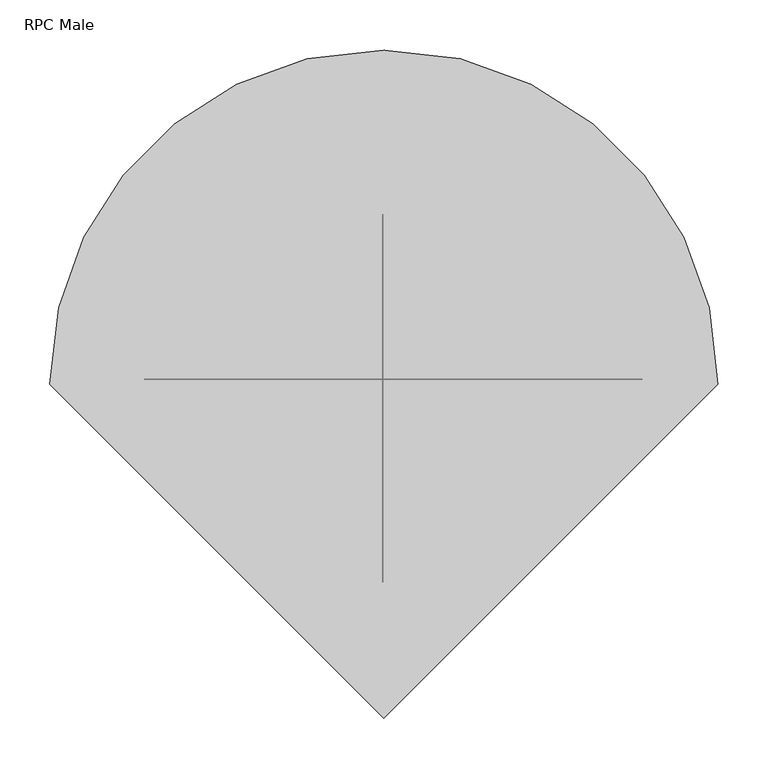
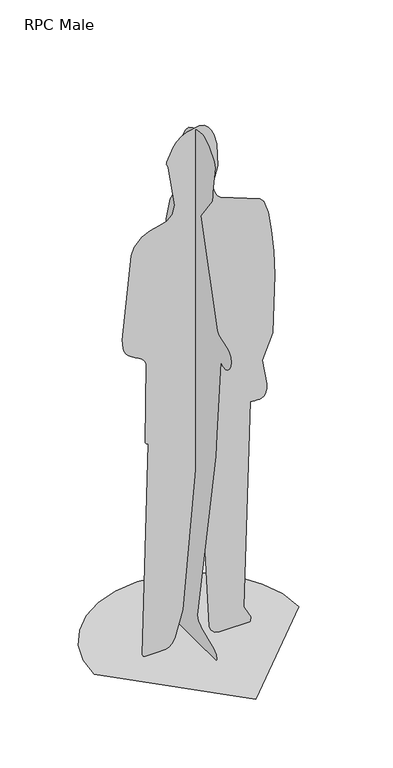
"""IFC4 building model written with IfcOpenShell, lengths in millimetres: proxy geometry, RPC Male : Dwayne."""

import ifcopenshell
import ifcopenshell.guid

model = None  # the IFC model being written
_history = None  # IfcOwnerHistory: only IFC2X3 demands one
_inside = {}  # id of a spatial element -> (the spatial element, [elements in it])
_under = {}  # id of a project, library or spatial element -> (it, [spatial elements below it])
_declared = {}  # id of a project -> (the project, [libraries it declares])
_typed = {}  # id of a type object -> (the type object, [elements of that type])
_made_of = {}  # id of a material, layer set ... -> (it, [elements and type objects made of it])


def new_model(schema):
    """Start an empty IFC model of exactly this schema.

    Asked for "IFC4X3", IfcOpenShell would pick the latest addendum, in which some entities
    have other attributes; the version numbers below select the first issue.
    IFC2X3 requires an IfcOwnerHistory on every rooted entity: one is made here for all.
    """
    global model, _history
    if schema == "IFC4X3":
        model = ifcopenshell.file(schema_version=(4, 3, 0, 0))
    else:
        model = ifcopenshell.file(schema=schema)
    _inside.clear()
    _under.clear()
    _declared.clear()
    _typed.clear()
    _made_of.clear()
    _history = None
    if model.schema == "IFC2X3":
        org = make("IfcOrganization", Name="unknown")
        user = make(
            "IfcPersonAndOrganization",
            ThePerson=make("IfcPerson", FamilyName="unknown"),
            TheOrganization=org,
        )
        app = make(
            "IfcApplication",
            ApplicationDeveloper=org,
            Version="unknown",
            ApplicationFullName="unknown",
            ApplicationIdentifier="unknown",
        )
        _history = make(
            "IfcOwnerHistory",
            OwningUser=user,
            OwningApplication=app,
            ChangeAction="ADDED",
            CreationDate=0,
        )
    return model


def make(cls, **values):
    """One entity of the class cls with the attributes given. An attribute that is None is left unset."""
    return model.create_entity(
        cls, **{name: value for name, value in values.items() if value is not None}
    )


def rooted(cls, **values):
    """An entity with a GlobalId (a new one), such as an element, a storey or a relation."""
    return make(cls, GlobalId=ifcopenshell.guid.new(), OwnerHistory=_history, **values)


def si_unit(unit_type, name, prefix=None):
    """IfcSIUnit, for example si_unit("LENGTHUNIT", "METRE", prefix="MILLI")."""
    return make("IfcSIUnit", UnitType=unit_type, Prefix=prefix, Name=name)


def assignment(units):
    """IfcUnitAssignment: the units of a project."""
    return None if units is None else make("IfcUnitAssignment", Units=units)


def point(xyz):
    """IfcCartesianPoint."""
    return None if xyz is None else make("IfcCartesianPoint", Coordinates=xyz)


def direction(xyz):
    """IfcDirection."""
    return None if xyz is None else make("IfcDirection", DirectionRatios=xyz)


def frame(location, z_axis=None, x_axis=None):
    """IfcAxis2Placement3D, a coordinate frame: its origin and axes. An axis left out is left unset."""
    return make(
        "IfcAxis2Placement3D",
        Location=point(location),
        Axis=direction(z_axis),
        RefDirection=direction(x_axis),
    )


def origin():
    """The frame at (0, 0, 0) with its axes left unset."""
    return frame((0.0, 0.0, 0.0))


def place(relative_to, where):
    """IfcLocalPlacement: puts the frame where relative to a parent placement (None: the world)."""
    return make(
        "IfcLocalPlacement", PlacementRelTo=relative_to, RelativePlacement=where
    )


def context(
    kind, dimensions, precision=None, world=None, true_north=None, identifier=None
):
    """IfcGeometricRepresentationContext, for example the 3D "Model" context."""
    return make(
        "IfcGeometricRepresentationContext",
        ContextIdentifier=identifier,
        ContextType=kind,
        CoordinateSpaceDimension=dimensions,
        Precision=precision,
        WorldCoordinateSystem=world,
        TrueNorth=true_north,
    )


def project(units=None, contexts=None):
    """IfcProject with its units and contexts."""
    return rooted(
        "IfcProject",
        Name="project",
        RepresentationContexts=contexts,
        UnitsInContext=assignment(units),
    )


def spatial(cls, under=None, at=None, **own):
    """A site, building, storey or space (cls), placed at a placement, below another one or the project."""
    s = rooted(cls, ObjectPlacement=at, **own)
    if under is not None:
        _under.setdefault(under.id(), (under, []))[1].append(s)
    return s


def point_list(points):
    """IfcCartesianPointList2D or 3D."""
    cls = (
        "IfcCartesianPointList2D" if len(points[0]) == 2 else "IfcCartesianPointList3D"
    )
    return make(cls, CoordList=points)


def triangles(points, corners, closed=None, point_numbers=None):
    """IfcTriangulatedFaceSet: each triangle names its three corners, points numbered from 1."""
    return make(
        "IfcTriangulatedFaceSet",
        Coordinates=point_list(points),
        Closed=closed,
        CoordIndex=corners,
        PnIndex=point_numbers,
    )


def shape(context_of_items, identifier, shape_type, items):
    """IfcShapeRepresentation: the items that make up one representation, for example the "Body"."""
    return make(
        "IfcShapeRepresentation",
        ContextOfItems=context_of_items,
        RepresentationIdentifier=identifier,
        RepresentationType=shape_type,
        Items=items,
    )


def source(mapping_origin, context_of_items, identifier, shape_type, items):
    """IfcRepresentationMap: a shape defined once, which mapped items show again and again."""
    return make(
        "IfcRepresentationMap",
        MappingOrigin=mapping_origin,
        MappedRepresentation=shape(context_of_items, identifier, shape_type, items),
    )


def transform(
    local_origin,
    x_axis=None,
    y_axis=None,
    z_axis=None,
    scale=None,
    scale2=None,
    scale3=None,
    uniform=True,
):
    """IfcCartesianTransformationOperator3D, or its non-uniform kind. x_axis, y_axis, z_axis: its Axis1, 2, 3."""
    if uniform:
        return make(
            "IfcCartesianTransformationOperator3D",
            Axis1=direction(x_axis),
            Axis2=direction(y_axis),
            LocalOrigin=point(local_origin),
            Scale=scale,
            Axis3=direction(z_axis),
        )
    return make(
        "IfcCartesianTransformationOperator3DnonUniform",
        Axis1=direction(x_axis),
        Axis2=direction(y_axis),
        LocalOrigin=point(local_origin),
        Scale=scale,
        Axis3=direction(z_axis),
        Scale2=scale2,
        Scale3=scale3,
    )


def mapped(mapping_source, mapping_target):
    """IfcMappedItem: shows the shape of a source again, moved by a transform."""
    return make(
        "IfcMappedItem", MappingSource=mapping_source, MappingTarget=mapping_target
    )


def made_of(thing, what):
    """Note that an element or type object is made of a material, layer set ...; save() writes the relation."""
    if what is not None:
        _made_of.setdefault(what.id(), (what, []))[1].append(thing)
    return thing


def element(
    cls,
    number,
    at=None,
    inside=None,
    cuts=None,
    type_object=None,
    material=None,
    context=None,
    identifier="Body",
    shape_type=None,
    held_by="IfcProductDefinitionShape",
    body=None,
    shapes=None,
    **own,
):
    """One element of the class cls, such as IfcWall. Its Tag is "e" and its number.

    at: its placement. inside: the storey or other place that contains it. cuts: it is an
    opening in that element (IfcRelVoidsElement). A single representation is given by context,
    identifier, shape_type and body (its items); several are given by shapes. held_by: the class
    of the entity that holds the representations. save() writes the other relations.
    """
    e = rooted(cls, Tag="e%d" % number, ObjectPlacement=at, **own)
    if body is not None:
        shapes = [shape(context, identifier, shape_type, body)]
    if shapes is not None:
        e.Representation = make(held_by, Representations=shapes)
    if inside is not None:
        _inside.setdefault(inside.id(), (inside, []))[1].append(e)
    if cuts is not None:
        rooted(
            "IfcRelVoidsElement", RelatingBuildingElement=cuts, RelatedOpeningElement=e
        )
    if type_object is not None:
        _typed.setdefault(type_object.id(), (type_object, []))[1].append(e)
    return made_of(e, material)


def aggregate(whole, parts):
    """IfcRelAggregates: a whole, such as a stair, and the parts it consists of."""
    return rooted("IfcRelAggregates", RelatingObject=whole, RelatedObjects=parts)


def save(model, path):
    """Write the relations noted so far, then the file.

    IfcRelAggregates (storeys below a building ...), IfcRelContainedInSpatialStructure (elements
    in a storey), IfcRelDefinesByType, IfcRelAssociatesMaterial and IfcRelDeclares: one each for
    every whole, place, type object, material and project.
    """
    for whole, parts in _under.values():
        aggregate(whole, parts)
    for where, things in _inside.values():
        rooted(
            "IfcRelContainedInSpatialStructure",
            RelatedElements=things,
            RelatingStructure=where,
        )
    for kind, things in _typed.values():
        rooted("IfcRelDefinesByType", RelatedObjects=things, RelatingType=kind)
    for what, things in _made_of.values():
        rooted("IfcRelAssociatesMaterial", RelatedObjects=things, RelatingMaterial=what)
    for by, libraries in _declared.values():
        rooted("IfcRelDeclares", RelatingContext=by, RelatedDefinitions=libraries)
    model.write(path)


def rpc_male_b6464c39(model_context):
    return source(origin(), model_context, "Body", "Tessellation", [
        triangles([(-180.7519758, 4.45e-05, 5.61e-05), (-184.2427693, 8.8e-06, 2.7953145), (-186.1721755, -1.66e-05, 5.8375002), (-186.8316374, -3.35e-05, 9.127569), (-168.2846227, -8.5e-06, 733.0652109), (-173.8813015, -8.5e-06, 735.2240908), (-177.6698602, -8.1e-06, 740.93319), (-174.1985423, 8.1e-06, 1013.6682867), (-179.591309, 8.8e-06, 1024.1651751), (-188.0395216, 9.6e-06, 1032.7759867), (-198.5267085, 9.9e-06, 1040.1126028), (-210.0363257, 1.03e-05, 1046.7864687), (-221.5520472, 1.07e-05, 1053.4092476), (-232.0572199, 1.1e-05, 1060.5929661), (-240.5353907, 1.14e-05, 1068.9488514), (-245.9518842, 1.21e-05, 1078.9880642), (-249.7386988, 1.29e-05, 1091.9821838), (-252.1552483, 1.4e-05, 1106.9298906), (-253.4607645, 1.47e-05, 1122.8295742), (-224.2188539, 3.16e-05, 1405.054644), (-213.7949444, 3.31e-05, 1430.2019463), (-189.1319694, 3.46e-05, 1456.0842327), (-160.624934, 3.53e-05, 1468.8737137), (-131.9229886, 3.57e-05, 1475.6378357), (-106.6752928, 3.64e-05, 1483.4436092), (-88.5310242, 3.71e-05, 1499.3593529), (-81.1392697, 3.9e-05, 1530.4516411), (-102.942045, 4.71e-05, 1666.4696468), (-107.9472446, 4.78e-05, 1679.2650867), (-108.1474504, 4.82e-05, 1680.5741638), (-107.984815, 4.82e-05, 1682.7587688), (-107.5268306, 4.82e-05, 1685.5190655), (-106.840944, 4.86e-05, 1688.5553627), (-86.6409052, 5.11e-05, 1733.0902897), (-74.2774293, 5.19e-05, 1747.7183212), (-59.5121605, 5.26e-05, 1759.6594528), (-42.363121, 5.33e-05, 1768.7777916), (-0.9855255, 5.37e-05, 1777.9990311), (15.8808757, 5.33e-05, 1772.5528519), (29.1619555, 5.26e-05, 1761.5639877), (39.2640369, 5.19e-05, 1747.0962662), (46.5934632, 5.08e-05, 1731.2140961), (56.009163, 4.89e-05, 1695.7207684), (59.1639487, 4.41e-05, 1618.2087845), (44.4858339, 4.12e-05, 1564.7278919), (44.3096682, 4.05e-05, 1551.1862766), (46.5532813, 3.94e-05, 1537.9279289), (51.2886345, 3.86e-05, 1525.4359589), (58.5876575, 3.83e-05, 1514.1926044), (68.5223164, 3.75e-05, 1504.6808304), (198.4030241, 3.46e-05, 1454.5808361), (210.7095586, 3.38e-05, 1440.8296406), (224.9005892, 3.13e-05, 1397.8447643), (235.5369131, 2.72e-05, 1333.6069702), (242.7580384, 2.28e-05, 1256.1532677), (246.7032373, 1.77e-05, 1173.5211021), (240.2781571, 5.9e-06, 974.9290089), (206.081389, 1.1e-06, 891.6222479), (221.1961823, -4e-06, 805.6633232), (220.4650678, -5.1e-06, 788.6200321), (214.9948893, -6.3e-06, 771.8045614), (210.3552016, -6.6e-06, 765.7300776), (204.1668257, -6.6e-06, 762.0919275), (196.8959759, -7e-06, 760.3982082), (189.0090118, -7e-06, 760.1573799), (180.9721295, -7e-06, 760.8774668), (173.2515615, -6.6e-06, 762.0669291), (166.3135766, -6.6e-06, 763.2339363), (144.8011179, -4.49e-05, 59.4752896), (168.6275342, -4.74e-05, 15.3365843), (166.1985945, 4.45e-05, 5.61e-05), (66.1332089, 4.45e-05, 5.61e-05), (49.8425018, 1.03e-05, 3.9765591), (39.0246256, -1.36e-05, 14.0353), (32.5983009, -2.91e-05, 28.3297116), (-2.7441046, -9.2e-06, 720.0458748), (-54.0725034, -1.03e-05, 117.9433278), (-81.3720135, 2.13e-05, 28.0047427), (-85.5237041, 2.69e-05, 19.9172686), (-91.2433859, 3.27e-05, 12.5691172), (-99.2451413, 3.86e-05, 5.9378887), (-110.2431982, 4.45e-05, 5.61e-05), (-13.8237406, 127.6718764, 9.9621145), (-13.8237974, 127.2617633, 182.0842528), (-13.8237815, 135.2635732, 744.8695776), (-13.8237815, 136.4149928, 748.3460369), (-13.8237815, 139.3954704, 752.5736132), (-13.8237815, 143.4944026, 757.5058702), (-13.8237815, 148.0010861, 763.0962994), (-13.8237815, 152.2049901, 769.2983917), (-13.8237792, 155.3953659, 776.0656385), (-13.8237792, 156.8616281, 783.3516764), (-13.8237622, 165.9465024, 1358.6137287), (-13.8237599, 143.2743216, 1442.0927902), (-13.8237576, 71.1145501, 1552.8585583), (-13.8237576, 64.3401725, 1580.5206779), (-13.8237542, 73.5344014, 1684.7952724), (-13.8237531, 67.2131212, 1712.2161278), (-13.8237531, 55.241223, 1734.9070393), (-13.8237531, 37.9260212, 1752.7537697), (-13.8237531, 15.5748771, 1765.6426632), (-13.8237531, -11.5049084, 1773.4593372), (-13.8237531, -43.0059914, 1776.090136), (-13.8237531, -55.0860226, 1772.9164925), (-13.8237542, -79.7038559, 1756.3218658), (-13.8237554, -107.4896145, 1722.3477768), (-13.8237554, -111.5711695, 1713.01012), (-13.8237554, -112.2229284, 1702.3019073), (-13.8237588, -99.0832235, 1611.9284992), (-13.8237588, -100.6007272, 1597.8206394), (-13.8237599, -96.755177, 1579.0656796), (-13.8237622, -31.1784566, 1488.4592915), (-13.8237735, -125.7984261, 1146.7472277), (-13.8237735, -134.1993577, 1137.675107), (-13.8237747, -184.2799037, 1119.3925747), (-13.8237747, -194.4649651, 1111.9394686), (-13.8237747, -201.1343255, 1100.3801451), (-13.8237769, -203.5508567, 1084.2058416), (-13.8237769, -200.9674025, 1068.9640394), (-13.8237769, -194.2820729, 1055.8707253), (-13.8237769, -184.3928146, 1046.1415226), (-13.8237769, -172.1978105, 1040.992709), (-13.8237769, -158.595007, 1041.6399078), (-13.8237769, -144.48246, 1049.299106), (-13.8237838, -123.0429529, 785.7648285), (-13.823786, -116.906318, 707.2429499), (-13.8237928, -10.2023683, 90.6853168), (-13.823794, -17.983895, 76.1481908), (-13.8237951, -35.4714404, 63.806743), (-13.8238042, -104.5965316, 31.8661463), (-13.8238053, -119.3344402, 20.2173661), (-13.8238076, -122.9915025, 6.7192091), (-13.8238042, -122.0607091, 4.3674998), (-13.8237894, -120.3451706, 2.3141478), (-13.8237724, -119.1853577, 1.4285653), (-13.8237474, -117.8199432, 0.6534771), (-13.8237099, -116.2458387, 5.61e-05), (-13.8237077, 124.501612, 0.0), (-348.4734607, -4.7230039, 0.0001684), (-339.5987117, 72.1961519, 0.0001684), (-314.3237646, 142.8340959, 5.61e-05), (-274.6722241, 205.1669827, 5.61e-05), (-222.6681673, 257.171094, 5.61e-05), (-160.3352533, 296.8225073, 5.61e-05), (-89.6973139, 322.097527, 5.61e-05), (-12.7781649, 330.972276, 5.61e-05), (64.1409886, 322.0975634, 5.61e-05), (134.7789371, 296.8225618, 5.61e-05), (197.1118239, 257.1710577, 5.61e-05), (249.1159897, 205.1670008, 5.61e-05), (288.7673667, 142.8340595, 5.61e-05), (314.0423864, 72.1960974, 0.0001684), (322.9171354, -4.7230331, 0.0001684), (-12.7782239, -340.4182474, 0.0001684)], [[71, 70, 72], [70, 69, 72], [72, 69, 73], [73, 69, 74], [74, 69, 75], [75, 69, 76], [69, 68, 76], [1, 82, 2], [2, 82, 3], [3, 82, 4], [82, 81, 4], [81, 80, 4], [80, 79, 4], [79, 78, 4], [78, 77, 4], [4, 77, 5], [77, 76, 5], [6, 5, 7], [5, 76, 7], [7, 76, 8], [76, 68, 8], [68, 67, 8], [67, 66, 8], [66, 65, 8], [65, 64, 8], [64, 63, 8], [63, 62, 8], [62, 61, 8], [61, 60, 8], [60, 59, 8], [59, 58, 8], [58, 57, 8], [57, 56, 8], [8, 56, 9], [56, 55, 9], [9, 55, 10], [55, 54, 10], [10, 54, 11], [54, 53, 11], [11, 53, 12], [53, 52, 12], [52, 51, 12], [51, 50, 12], [12, 50, 13], [13, 50, 14], [14, 50, 15], [15, 50, 16], [16, 50, 17], [17, 50, 18], [18, 50, 19], [19, 50, 20], [20, 50, 21], [21, 50, 22], [22, 50, 23], [23, 50, 24], [24, 50, 25], [25, 50, 26], [50, 49, 26], [49, 48, 26], [26, 48, 27], [48, 47, 27], [47, 46, 27], [46, 45, 27], [45, 44, 27], [27, 44, 28], [44, 43, 28], [43, 42, 28], [28, 42, 29], [29, 42, 30], [30, 42, 31], [31, 42, 32], [32, 42, 33], [33, 42, 34], [34, 42, 35], [35, 42, 36], [36, 42, 37], [42, 41, 37], [41, 40, 37], [37, 40, 38], [38, 40, 39], [138, 137, 83], [83, 137, 84], [137, 136, 84], [136, 135, 84], [131, 130, 132], [132, 130, 133], [133, 130, 134], [134, 130, 135], [123, 122, 124], [122, 121, 124], [121, 120, 124], [120, 119, 124], [119, 118, 124], [118, 117, 124], [117, 116, 124], [116, 115, 124], [115, 114, 124], [114, 113, 124], [107, 106, 108], [106, 105, 108], [105, 104, 108], [104, 103, 108], [103, 102, 108], [102, 101, 108], [101, 100, 108], [100, 99, 108], [99, 98, 108], [98, 97, 108], [108, 97, 109], [109, 97, 110], [110, 97, 111], [97, 96, 111], [96, 95, 111], [111, 95, 112], [95, 94, 112], [94, 93, 112], [112, 93, 113], [93, 92, 113], [113, 92, 124], [124, 92, 125], [92, 91, 125], [91, 90, 125], [90, 89, 125], [89, 88, 125], [88, 87, 125], [87, 86, 125], [125, 86, 126], [86, 85, 126], [126, 85, 127], [85, 84, 127], [127, 84, 128], [84, 135, 128], [128, 135, 129], [135, 130, 129], [154, 153, 139], [153, 152, 139], [139, 152, 140], [152, 151, 140], [140, 151, 141], [141, 151, 142], [151, 150, 142], [150, 149, 142], [142, 149, 143], [143, 149, 144], [144, 149, 145], [145, 149, 146], [146, 149, 147], [147, 149, 148]], closed=False),
    ])


if __name__ == "__main__":
    model = new_model("IFC4")
    model_context = context("Model", 3, world=origin())
    ifc_project = project(units=[si_unit("LENGTHUNIT", "METRE", prefix="MILLI")], contexts=[model_context])
    site = spatial("IfcSite", under=ifc_project)
    building = spatial("IfcBuilding", under=site)
    placement = place(None, origin())
    rpc_male_shape = rpc_male_b6464c39(model_context)
    element("IfcBuildingElementProxy", 1, Name="RPC Male : Dwayne", ObjectType="RPC Male : Dwayne", at=placement, inside=building, context=model_context, shape_type="MappedRepresentation", body=[
        mapped(rpc_male_shape, transform((0.0, 0.0, 0.0), x_axis=(1.0, 0.0, 0.0), y_axis=(0.0, 1.0, 0.0), z_axis=(0.0, 0.0, 1.0))),
    ])
    save(model, "model.ifc")

# Revit data of these elements
# Type "RPC Male : Dwayne"
#   built-in parameter 1005198 = "{2, 15},{22, RPC-8-G1AE-S4G0-CKUK-A},{1, 0},{1, 0},{2, 15},{1, 8},{5, Color},{1, 0},{1, 0},{3, 0.8},{3, 0.8},{3, 0.8},{1, 8},{7, BBoxMin},{1, 0},{1, 0},{1, 0},{1, 0},{1, 0},{1, 8},{7, BBoxMax},{1, 0},{1, 0},{1, 0},{1, 0},{1, 0},{2, 11},{9, RPCTypeId},{1, 0},{1, 0},{22, RPC-8-G1AE-S4G0-CKUK-A},{1, 6},{14, RPCPlantHeight},{1, 0},{1, 0},{7, 5.83333},{2, 11},{7, keyword},{1, 0},{1, 0},{45, :RPCs:People [Business-Hispanic]:Geometry:RPC},{2, 11},{8, category},{1, 0},{1, 0},{26, People [Business-Hispanic]},{2, 11},{12, LocalizedUID},{1, 0},{1, 0},{6, Dwayne},{2, 14},{6, Height},{1, 0},{1, 0},{7, 5.83333},{1, 2},{16, Cast Reflections},{1, 0},{1, 0},{1, 0},{1, 2},{6, Jitter},{1, 0},{1, 0},{1, 1},{1, 2},{9, Billboard},{1, 0},{1, 0},{1, 0},{1, 2},{12, Cast Shadows},{1, 0},{1, 0},{1, 1},{1, 2},{20, Apply Filter Effects},{1, 0},{1, 0},{1, 0},{2, 11},{28, Apply Filter Effects-Text-FC},{1, 0},{1, 0},{4, None},{21, assetlibrary_base.fbx},{1, 5},"
#   built-in parameter 1005195 = "RPC-8-G1AE-S4G0-CKUK-A"
#   Height = 0
